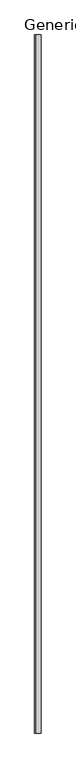
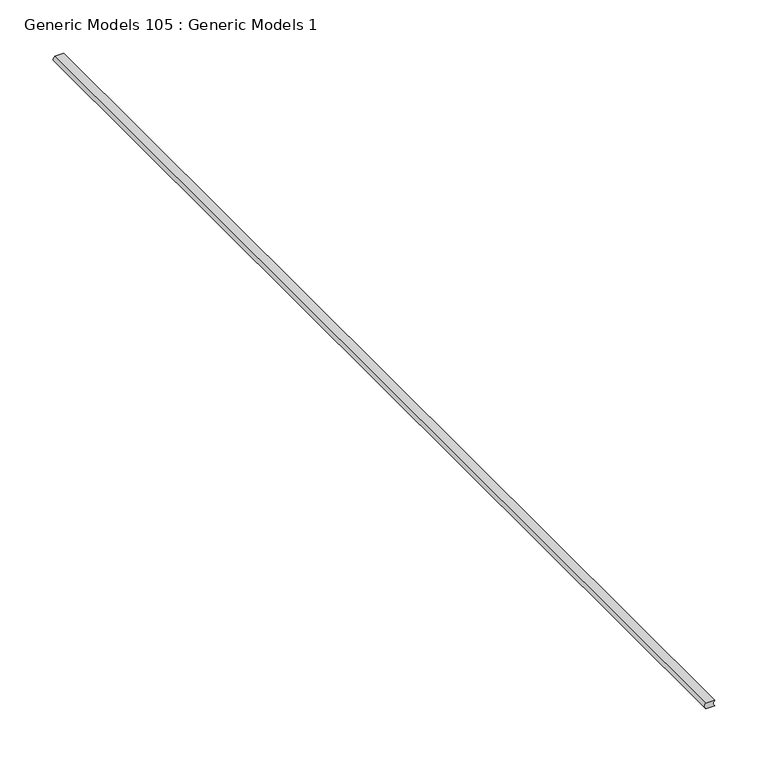
"""IFC4 building model written with IfcOpenShell, lengths in millimetres: proxy geometry, Generic Models 105 : Generic Models 1."""

from ifc_helpers import new_model, si_unit, point, frame, frame_2d, origin, place, context, project, spatial, polyline, circle_curve, trimmed, segment, composite_curve, outline, extrude, source, transform, mapped, element, save


def generic_models_105_generic_models_1_4289aad1(model_context):
    return source(origin(), model_context, "Body", "SweptSolid", [
        extrude(outline(composite_curve([segment(trimmed(circle_curve(frame_2d((3.175, 51021.9897405)), 4.3100275), [point((0.0, 51019.075))], [point((6.35, 51019.075))], True, "CARTESIAN"), True, "CONTINUOUS"), segment(polyline([(6.35, 51019.075), (6.35, 51009.55)]), True, "CONTINUOUS"), segment(trimmed(circle_curve(frame_2d((3.175, 51012.4647405)), 4.3100275), [point((6.35, 51009.55))], [point((0.0, 51009.55))], False, "CARTESIAN"), True, "CONTINUOUS"), segment(polyline([(0.0, 51009.55), (0.0, 51019.075)]), True, "CONTINUOUS")], self_intersect=False)), frame((0.0, 0.0, 0.0), z_axis=(0.0, 1.0, 0.0), x_axis=(0.0, 0.0, 1.0)), (0.0, 0.0, 1.0), 1219.2),
    ])


if __name__ == "__main__":
    model = new_model("IFC4")
    model_context = context("Model", 3, world=origin())
    ifc_project = project(units=[si_unit("LENGTHUNIT", "METRE", prefix="MILLI")], contexts=[model_context])
    site = spatial("IfcSite", under=ifc_project)
    building = spatial("IfcBuilding", under=site)
    placement = place(None, origin())
    generic_models_105_generic_models_1_shape = generic_models_105_generic_models_1_4289aad1(model_context)
    element("IfcBuildingElementProxy", 1, Name="Generic Models 105 : Generic Models 1", ObjectType="Generic Models 105 : Generic Models 1", at=placement, inside=building, context=model_context, shape_type="MappedRepresentation", body=[
        mapped(generic_models_105_generic_models_1_shape, transform((0.0, 0.0, 0.0), x_axis=(1.0, 0.0, 0.0), y_axis=(0.0, 1.0, 0.0), z_axis=(0.0, 0.0, 1.0))),
    ])
    save(model, "model.ifc")

# Revit data of these elements
# Element 1 (IfcBuildingElementProxy, "Generic Models 105 : Generic Models 1")
#   Materials on its faces: "ACOUSTICAL SEALANT"
# Materials
#   "ACOUSTICAL SEALANT": class "Unassigned", colour RGB 120 120 120, transparency 0, Cost = 0
